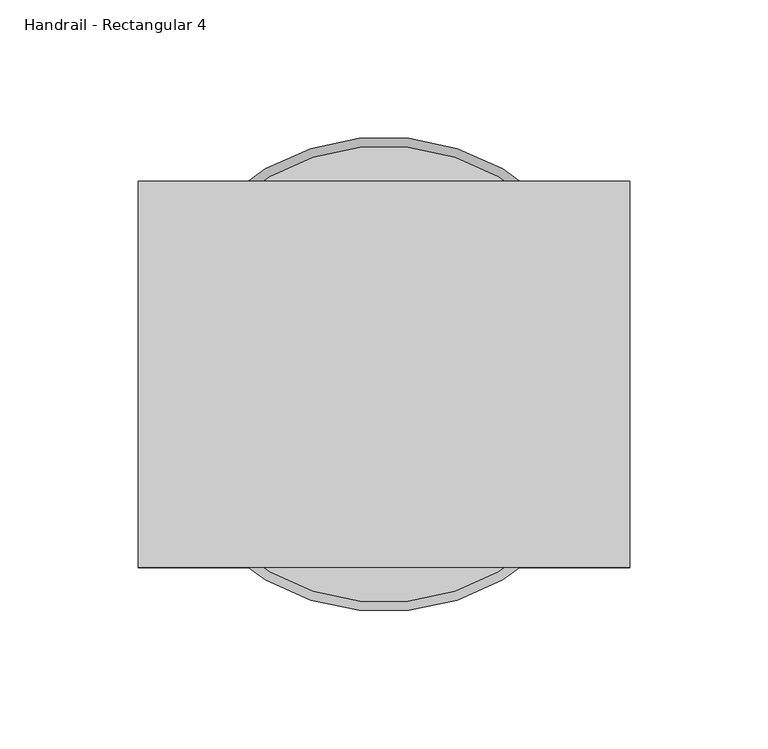
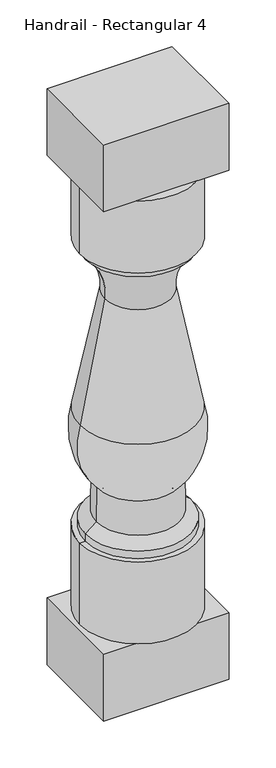
"""IFC4 building model written with IfcOpenShell, lengths in millimetres: railing geometry, Handrail - Rectangular 4."""

from ifc_helpers import new_model, si_unit, point, frame, origin, place, context, project, spatial, polyline, circle_curve, ellipse_curve, trimmed, outline, extrude, source, transform, mapped, element, save
from ifc_brep_helpers import plane_surface, cylinder_surface, revolved_surface, advanced_brep


def handrail_rectangular_4_9431a996(model_context):
    return source(origin(), model_context, "Body", "SolidModel", [
        advanced_brep(
        [(13846.7021895, -1665.6164768, 874.7125), (14011.8021895, -1665.6164768, 874.7125), (13929.2521895, -1665.6164768, 874.7125), (13846.7021895, -1665.6164768, 766.7625), (14011.8021895, -1665.6164768, 766.7625), (13854.6396895, -1665.6164768, 766.7625), (14003.8646895, -1665.6164768, 766.7625), (13854.6396895, -1665.6164768, 755.65), (14003.8646895, -1665.6164768, 755.65), (13882.4209395, -1665.6164768, 687.3875), (13976.0834395, -1665.6164768, 687.3875), (13847.4959395, -1665.6164768, 509.5875), (14011.0084395, -1665.6164768, 509.5875), (13871.3084395, -1665.6164768, 407.9875), (13987.1959395, -1665.6164768, 407.9875), (13870.5146895, -1665.6164768, 357.1875), (13987.9896895, -1665.6164768, 357.1875), (13854.6396895, -1665.6164768, 344.4875), (14003.8646895, -1665.6164768, 344.4875), (13854.6396895, -1665.6164768, 333.375), (14003.8646895, -1665.6164768, 333.375), (13846.7021895, -1665.6164768, 333.375), (14011.8021895, -1665.6164768, 333.375), (13846.7021895, -1665.6164768, 211.1375), (14011.8021895, -1665.6164768, 211.1375), (13929.2521895, -1665.6164768, 211.1375)],
        [
            (0, 1, circle_curve(frame((13929.2521895, -1665.6164768, 874.7125), z_axis=(0.0, 0.0, 1.0), x_axis=(1.0, 0.0, 0.0)), 82.55)),
            (1, 2),
            (2, 0),
            (1, 0, circle_curve(frame((13929.2521895, -1665.6164768, 874.7125), z_axis=(0.0, 0.0, 1.0), x_axis=(1.0, 0.0, 0.0)), 82.55)),
            (3, 4, circle_curve(frame((13929.2521895, -1665.6164768, 766.7625), z_axis=(0.0, 0.0, 1.0), x_axis=(1.0, 0.0, 0.0)), 82.55)),
            (4, 1),
            (0, 3),
            (4, 3, circle_curve(frame((13929.2521895, -1665.6164768, 766.7625), z_axis=(0.0, 0.0, 1.0), x_axis=(1.0, 0.0, 0.0)), 82.55)),
            (5, 6, circle_curve(frame((13929.2521895, -1665.6164768, 766.7625), z_axis=(0.0, 0.0, 1.0), x_axis=(1.0, 0.0, 0.0)), 74.6125)),
            (6, 4),
            (3, 5),
            (6, 5, circle_curve(frame((13929.2521895, -1665.6164768, 766.7625), z_axis=(0.0, 0.0, 1.0), x_axis=(1.0, 0.0, 0.0)), 74.6125)),
            (7, 8, circle_curve(frame((13929.2521895, -1665.6164768, 755.65), z_axis=(0.0, 0.0, 1.0), x_axis=(1.0, 0.0, 0.0)), 74.6125)),
            (8, 6),
            (5, 7),
            (8, 7, circle_curve(frame((13929.2521895, -1665.6164768, 755.65), z_axis=(0.0, 0.0, 1.0), x_axis=(1.0, 0.0, 0.0)), 74.6125)),
            (9, 10, circle_curve(frame((13929.2521895, -1665.6164768, 687.3875), z_axis=(0.0, 0.0, 1.0), x_axis=(1.0, 0.0, 0.0)), 46.83125)),
            (10, 8, circle_curve(frame((14055.2574242, -1665.6164768, 694.9499409), z_axis=(0.0, 1.0, 0.0), x_axis=(-1.0, 0.0, 0.0)), 79.5343344)),
            (7, 9, circle_curve(frame((13803.2469549, -1665.6164768, 694.9499409), z_axis=(0.0, 1.0, 0.0), x_axis=(1.0, 0.0, 0.0)), 79.5343344)),
            (10, 9, circle_curve(frame((13929.2521895, -1665.6164768, 687.3875), z_axis=(0.0, 0.0, 1.0), x_axis=(1.0, 0.0, 0.0)), 46.83125)),
            (11, 12, circle_curve(frame((13929.2521895, -1665.6164768, 509.5875), z_axis=(0.0, 0.0, 1.0), x_axis=(1.0, 0.0, 0.0)), 81.75625)),
            (12, 10, circle_curve(frame((14891.0418945, -1665.6164768, 774.7813483), z_axis=(0.0, 1.0, 0.0), x_axis=(-1.0, 0.0, 0.0)), 919.122766)),
            (9, 11, circle_curve(frame((12967.4624846, -1665.6164768, 774.7813483), z_axis=(0.0, 1.0, 0.0), x_axis=(1.0, 0.0, 0.0)), 919.122766)),
            (12, 11, circle_curve(frame((13929.2521895, -1665.6164768, 509.5875), z_axis=(0.0, 0.0, 1.0), x_axis=(1.0, 0.0, 0.0)), 81.75625)),
            (13, 14, circle_curve(frame((13929.2521895, -1665.6164768, 407.9875), z_axis=(0.0, 0.0, 1.0), x_axis=(1.0, 0.0, 0.0)), 57.94375)),
            (14, 12, circle_curve(frame((13910.9738909, -1665.6164768, 479.44257), z_axis=(0.0, -1.0, 0.0), x_axis=(-1.0, 0.0, 0.0)), 104.4778815)),
            (11, 13, circle_curve(frame((13947.5304882, -1665.6164768, 479.44257), z_axis=(0.0, -1.0, 0.0), x_axis=(1.0, 0.0, 0.0)), 104.4778815)),
            (14, 13, circle_curve(frame((13929.2521895, -1665.6164768, 407.9875), z_axis=(0.0, 0.0, 1.0), x_axis=(1.0, 0.0, 0.0)), 57.94375)),
            (15, 16, circle_curve(frame((13929.2521895, -1665.6164768, 357.1875), z_axis=(0.0, 0.0, 1.0), x_axis=(1.0, 0.0, 0.0)), 58.7375)),
            (16, 14),
            (13, 15),
            (16, 15, circle_curve(frame((13929.2521895, -1665.6164768, 357.1875), z_axis=(0.0, 0.0, 1.0), x_axis=(1.0, 0.0, 0.0)), 58.7375)),
            (17, 18, circle_curve(frame((13929.2521895, -1665.6164768, 344.4875), z_axis=(0.0, 0.0, 1.0), x_axis=(1.0, 0.0, 0.0)), 74.6125)),
            (18, 16),
            (15, 17),
            (18, 17, circle_curve(frame((13929.2521895, -1665.6164768, 344.4875), z_axis=(0.0, 0.0, 1.0), x_axis=(1.0, 0.0, 0.0)), 74.6125)),
            (19, 20, circle_curve(frame((13929.2521895, -1665.6164768, 333.375), z_axis=(0.0, 0.0, 1.0), x_axis=(1.0, 0.0, 0.0)), 74.6125)),
            (20, 18),
            (17, 19),
            (20, 19, circle_curve(frame((13929.2521895, -1665.6164768, 333.375), z_axis=(0.0, 0.0, 1.0), x_axis=(1.0, 0.0, 0.0)), 74.6125)),
            (21, 22, circle_curve(frame((13929.2521895, -1665.6164768, 333.375), z_axis=(0.0, 0.0, 1.0), x_axis=(1.0, 0.0, 0.0)), 82.55)),
            (22, 20),
            (19, 21),
            (22, 21, circle_curve(frame((13929.2521895, -1665.6164768, 333.375), z_axis=(0.0, 0.0, 1.0), x_axis=(1.0, 0.0, 0.0)), 82.55)),
            (23, 24, circle_curve(frame((13929.2521895, -1665.6164768, 211.1375), z_axis=(0.0, 0.0, 1.0), x_axis=(1.0, 0.0, 0.0)), 82.55)),
            (24, 22),
            (21, 23),
            (24, 23, circle_curve(frame((13929.2521895, -1665.6164768, 211.1375), z_axis=(0.0, 0.0, 1.0), x_axis=(1.0, 0.0, 0.0)), 82.55)),
            (25, 24),
            (23, 25),
        ],
        [
            plane_surface(frame((13929.2521895, -1665.6164768, 874.7125), z_axis=(0.0, 0.0, 1.0), x_axis=(1.0, 0.0, 0.0))),
            cylinder_surface(frame((13929.2521895, -1665.6164768, 839.7875), z_axis=(0.0, 0.0, -1.0), x_axis=(1.0, 0.0, 0.0)), 82.55),
            plane_surface(frame((13929.2521895, -1665.6164768, 766.7625), z_axis=(0.0, 0.0, -1.0), x_axis=(1.0, 0.0, 0.0))),
            cylinder_surface(frame((13929.2521895, -1665.6164768, 839.7875), z_axis=(0.0, 0.0, -1.0), x_axis=(1.0, 0.0, 0.0)), 74.6125),
            revolved_surface(trimmed(ellipse_curve(frame((14055.2574242, -1665.6164768, 694.9499409), z_axis=(0.0, -1.0, 0.0), x_axis=(-1.0, 0.0, 0.0)), 79.5343344, 79.5343344), [point((14003.8646895, -1665.6164768, 755.65))], [point((13976.0834395, -1665.6164768, 687.3875))], True, "CARTESIAN"), (13929.2521895, -1665.6164768, 839.7875), (0.0, 0.0, -1.0)),
            revolved_surface(trimmed(ellipse_curve(frame((14891.0418945, -1665.6164768, 774.7813483), z_axis=(0.0, -1.0, 0.0), x_axis=(-1.0, 0.0, 0.0)), 919.122766, 919.122766), [point((13976.0834395, -1665.6164768, 687.3875))], [point((14011.0084395, -1665.6164768, 509.5875))], True, "CARTESIAN"), (13929.2521895, -1665.6164768, 839.7875), (0.0, 0.0, -1.0)),
            revolved_surface(trimmed(ellipse_curve(frame((13910.9738909, -1665.6164768, 479.44257), z_axis=(0.0, 1.0, 0.0), x_axis=(-1.0, 0.0, 0.0)), 104.4778815, 104.4778815), [point((14011.0084395, -1665.6164768, 509.5875))], [point((13987.1959395, -1665.6164768, 407.9875))], True, "CARTESIAN"), (13929.2521895, -1665.6164768, 839.7875), (0.0, 0.0, -1.0)),
            revolved_surface(polyline([(13987.1959395, -1665.6164768, 407.9875), (13987.9896895, -1665.6164768, 357.1875)]), (13929.2521895, -1665.6164768, 839.7875), (0.0, 0.0, -1.0)),
            revolved_surface(polyline([(13987.9896895, -1665.6164768, 357.1875), (14003.8646895, -1665.6164768, 344.4875)]), (13929.2521895, -1665.6164768, 839.7875), (0.0, 0.0, -1.0)),
            plane_surface(frame((13929.2521895, -1665.6164768, 333.375), z_axis=(0.0, 0.0, 1.0), x_axis=(1.0, 0.0, 0.0))),
            plane_surface(frame((13929.2521895, -1665.6164768, 211.1375), z_axis=(0.0, 0.0, -1.0), x_axis=(1.0, 0.0, 0.0))),
        ],
        [
            (0, [[1, 2, 3]]),
            (0, [[4, -3, -2]]),
            (1, [[5, 6, -1, 7]]),
            (1, [[8, -7, -4, -6]]),
            (2, [[9, 10, -5, 11]]),
            (2, [[12, -11, -8, -10]]),
            (3, [[13, 14, -9, 15]]),
            (3, [[16, -15, -12, -14]]),
            (4, [[17, 18, -13, 19]]),
            (4, [[20, -19, -16, -18]]),
            (5, [[21, 22, -17, 23]]),
            (5, [[24, -23, -20, -22]]),
            (6, [[25, 26, -21, 27]]),
            (6, [[28, -27, -24, -26]]),
            (7, [[29, 30, -25, 31]]),
            (7, [[32, -31, -28, -30]]),
            (8, [[33, 34, -29, 35]]),
            (8, [[36, -35, -32, -34]]),
            (3, [[37, 38, -33, 39]]),
            (3, [[40, -39, -36, -38]]),
            (9, [[41, 42, -37, 43]]),
            (9, [[44, -43, -40, -42]]),
            (1, [[45, 46, -41, 47]]),
            (1, [[48, -47, -44, -46]]),
            (10, [[49, -45, 50]]),
            (10, [[-50, -48, -49]]),
        ],
    ),
        extrude(outline(polyline([(13840.3521895, -1735.4664768), (13840.3521895, -1595.7664768), (14018.1521895, -1595.7664768), (14018.1521895, -1735.4664768), (13840.3521895, -1735.4664768)])), frame((0.0, 0.0, 111.125), z_axis=(0.0, 0.0, 1.0), x_axis=(1.0, 0.0, 0.0)), (0.0, 0.0, 1.0), 100.0125),
        extrude(outline(polyline([(13840.3521895, -1595.7664768), (14018.1521895, -1595.7664768), (14018.1521895, -1735.4664768), (13840.3521895, -1735.4664768), (13840.3521895, -1595.7664768)])), frame((0.0, 0.0, 874.7125), z_axis=(0.0, 0.0, 1.0), x_axis=(1.0, 0.0, 0.0)), (0.0, 0.0, 1.0), 100.0125),
    ])


if __name__ == "__main__":
    model = new_model("IFC4")
    model_context = context("Model", 3, world=origin())
    ifc_project = project(units=[si_unit("LENGTHUNIT", "METRE", prefix="MILLI")], contexts=[model_context])
    site = spatial("IfcSite", under=ifc_project)
    building = spatial("IfcBuilding", under=site)
    placement = place(None, origin())
    handrail_rectangular_4_shape = handrail_rectangular_4_9431a996(model_context)
    element("IfcRailing", 1, ObjectType="Handrail - Rectangular 4", at=placement, inside=building, context=model_context, shape_type="MappedRepresentation", body=[
        mapped(handrail_rectangular_4_shape, transform((0.0, 0.0, 0.0), x_axis=(1.0, 0.0, 0.0), y_axis=(0.0, 1.0, 0.0), z_axis=(0.0, 0.0, 1.0))),
    ])
    save(model, "model.ifc")
